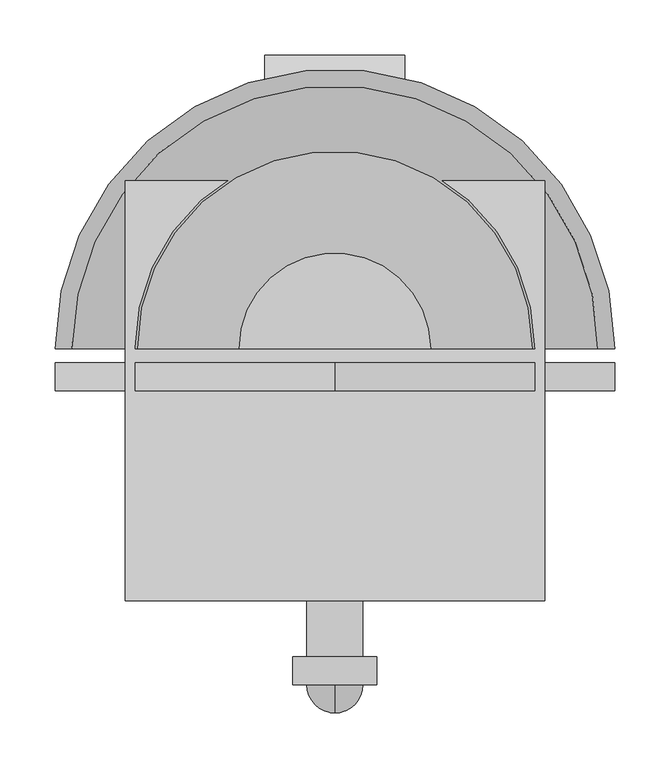
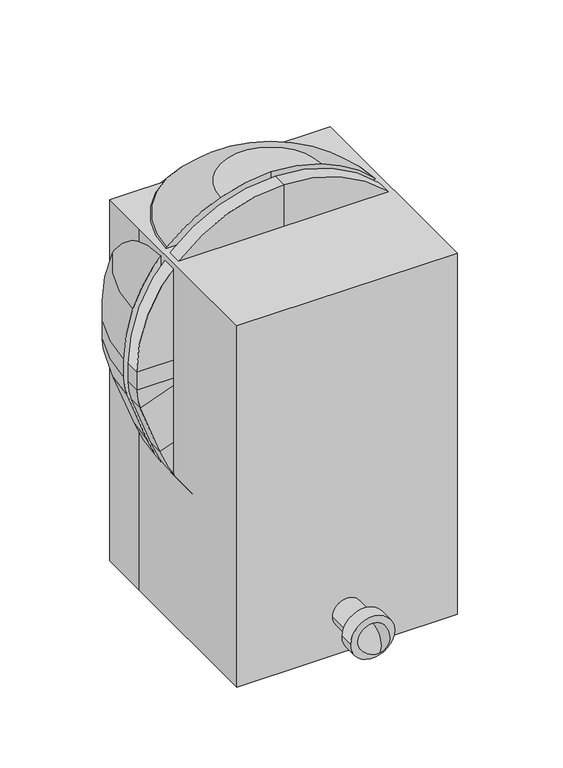
"""IFC4 building model written with IfcOpenShell, lengths in millimetres: proxy geometry, P9050 - Toilet, Wall Hung, Siphon Jet : P9050 - Toilet, Wall Hung, Siphon Jet."""

from ifc_helpers import new_model, si_unit, point, frame, frame_2d, origin, origin_with_axes, place, context, project, spatial, polyline, circle_curve, ellipse_curve, trimmed, segment, composite_curve, outline, extrude, source, transform, mapped, element, save
from ifc_brep_helpers import plane_surface, cylinder_surface, revolved_surface, advanced_brep


def specialty_equipment_177a83fe(model_context):
    return source(origin(), model_context, "Body", "SolidModel", [
        advanced_brep(
        [(-86.8731164, 38.1, 721.2819257), (-179.6051224, 38.1, 662.2051224), (-238.6819257, 38.1, 569.4731164), (-254.0, 38.1, 482.6), (-254.0, 38.1, 449.7148212), (-247.8727703, 38.1, 414.9655747), (-214.4568992, 38.1, 323.1562234), (-180.7778621, 38.1, 258.4593951), (-135.6735798, 38.1, 194.0438043), (-78.7437471, 38.1, 154.1811063), (0.0, 38.1, 133.0817829), (0.0, 38.1, 159.3777978), (-63.2399099, 38.1, 176.3228806), (-120.1697426, 38.1, 216.1855786), (-158.0533758, 38.1, 270.2890139), (-191.7324129, 38.1, 334.9858422), (-224.0045777, 38.1, 423.6528863), (-228.6, 38.1, 449.7148212), (-228.6, 38.1, 482.6), (-214.8137331, 38.1, 560.7858048), (-161.6446102, 38.1, 644.2446102), (-78.1858048, 38.1, 697.4137331), (0.0, 38.1, 711.2), (0.0, 38.1, 736.6), (86.8731164, 38.1, 721.2819257), (78.1858048, 38.1, 697.4137331), (161.6446102, 38.1, 644.2446102), (214.8137331, 38.1, 560.7858048), (228.6, 38.1, 482.6), (228.6, 38.1, 449.7148212), (224.0045777, 38.1, 423.6528863), (191.7324129, 38.1, 334.9858422), (158.0533758, 38.1, 270.2890139), (120.1697426, 38.1, 216.1855786), (63.2399099, 38.1, 176.3228806), (78.7437471, 38.1, 154.1811063), (135.6735798, 38.1, 194.0438043), (180.7778621, 38.1, 258.4593951), (214.4568992, 38.1, 323.1562234), (247.8727703, 38.1, 414.9655747), (254.0, 38.1, 449.7148212), (254.0, 38.1, 482.6), (238.6819257, 38.1, 569.4731164), (179.6051224, 38.1, 662.2051224)],
        [
            (0, 1, circle_curve(frame((0.0, 38.1, 482.6), z_axis=(0.0, -1.0, 0.0), x_axis=(-1.0, 0.0, 0.0)), 254.0)),
            (1, 2, circle_curve(frame((0.0, 38.1, 482.6), z_axis=(0.0, -1.0, 0.0), x_axis=(-1.0, 0.0, 0.0)), 254.0)),
            (2, 3, circle_curve(frame((0.0, 38.1, 482.6), z_axis=(0.0, -1.0, 0.0), x_axis=(-1.0, 0.0, 0.0)), 254.0)),
            (3, 4),
            (4, 5, circle_curve(frame((-152.4, 38.1, 449.7148212), z_axis=(0.0, -1.0, 0.0), x_axis=(-1.0, 0.0, 0.0)), 101.6)),
            (5, 6),
            (6, 7, circle_curve(frame((48.0932191, 38.1, 418.7166514), z_axis=(0.0, -1.0, 0.0), x_axis=(-1.0, 0.0, 0.0)), 279.4)),
            (7, 8),
            (8, 9, circle_curve(frame((-52.4477321, 38.1, 252.3191703), z_axis=(0.0, -1.0, 0.0), x_axis=(-1.0, 0.0, 0.0)), 101.6)),
            (9, 10),
            (10, 11),
            (11, 12),
            (12, 13, circle_curve(frame((-36.9438949, 38.1, 274.4609446), z_axis=(0.0, 1.0, 0.0), x_axis=(-1.0, 0.0, 0.0)), 101.6)),
            (13, 14),
            (14, 15, circle_curve(frame((70.8177054, 38.1, 430.5462703), z_axis=(0.0, 1.0, 0.0), x_axis=(-1.0, 0.0, 0.0)), 279.4)),
            (15, 16),
            (16, 17, circle_curve(frame((-152.4, 38.1, 449.7148212), z_axis=(0.0, 1.0, 0.0), x_axis=(-1.0, 0.0, 0.0)), 76.2)),
            (17, 18),
            (18, 19, circle_curve(frame((0.0, 38.1, 482.6), z_axis=(0.0, 1.0, 0.0), x_axis=(-1.0, 0.0, 0.0)), 228.6)),
            (19, 20, circle_curve(frame((0.0, 38.1, 482.6), z_axis=(0.0, 1.0, 0.0), x_axis=(-1.0, 0.0, 0.0)), 228.6)),
            (20, 21, circle_curve(frame((0.0, 38.1, 482.6), z_axis=(0.0, 1.0, 0.0), x_axis=(-1.0, 0.0, 0.0)), 228.6)),
            (21, 22, circle_curve(frame((0.0, 38.1, 482.6), z_axis=(0.0, 1.0, 0.0), x_axis=(-1.0, 0.0, 0.0)), 228.6)),
            (22, 23),
            (23, 0, circle_curve(frame((0.0, 38.1, 482.6), z_axis=(0.0, -1.0, 0.0), x_axis=(-1.0, 0.0, 0.0)), 254.0)),
            (24, 23, circle_curve(frame((0.0, 38.1, 482.6), z_axis=(0.0, -1.0, 0.0), x_axis=(1.0, 0.0, 0.0)), 254.0)),
            (22, 25, circle_curve(frame((0.0, 38.1, 482.6), z_axis=(0.0, 1.0, 0.0), x_axis=(1.0, 0.0, 0.0)), 228.6)),
            (25, 26, circle_curve(frame((0.0, 38.1, 482.6), z_axis=(0.0, 1.0, 0.0), x_axis=(1.0, 0.0, 0.0)), 228.6)),
            (26, 27, circle_curve(frame((0.0, 38.1, 482.6), z_axis=(0.0, 1.0, 0.0), x_axis=(1.0, 0.0, 0.0)), 228.6)),
            (27, 28, circle_curve(frame((0.0, 38.1, 482.6), z_axis=(0.0, 1.0, 0.0), x_axis=(1.0, 0.0, 0.0)), 228.6)),
            (28, 29),
            (29, 30, circle_curve(frame((152.4, 38.1, 449.7148212), z_axis=(0.0, 1.0, 0.0), x_axis=(1.0, 0.0, 0.0)), 76.2)),
            (30, 31),
            (31, 32, circle_curve(frame((-70.8177054, 38.1, 430.5462703), z_axis=(0.0, 1.0, 0.0), x_axis=(1.0, 0.0, 0.0)), 279.4)),
            (32, 33),
            (33, 34, circle_curve(frame((36.9438949, 38.1, 274.4609446), z_axis=(0.0, 1.0, 0.0), x_axis=(1.0, 0.0, 0.0)), 101.6)),
            (34, 11),
            (10, 35),
            (35, 36, circle_curve(frame((52.4477321, 38.1, 252.3191703), z_axis=(0.0, -1.0, 0.0), x_axis=(1.0, 0.0, 0.0)), 101.6)),
            (36, 37),
            (37, 38, circle_curve(frame((-48.0932191, 38.1, 418.7166514), z_axis=(0.0, -1.0, 0.0), x_axis=(1.0, 0.0, 0.0)), 279.4)),
            (38, 39),
            (39, 40, circle_curve(frame((152.4, 38.1, 449.7148212), z_axis=(0.0, -1.0, 0.0), x_axis=(1.0, 0.0, 0.0)), 101.6)),
            (40, 41),
            (41, 42, circle_curve(frame((0.0, 38.1, 482.6), z_axis=(0.0, -1.0, 0.0), x_axis=(1.0, 0.0, 0.0)), 254.0)),
            (42, 43, circle_curve(frame((0.0, 38.1, 482.6), z_axis=(0.0, -1.0, 0.0), x_axis=(1.0, 0.0, 0.0)), 254.0)),
            (43, 24, circle_curve(frame((0.0, 38.1, 482.6), z_axis=(0.0, -1.0, 0.0), x_axis=(1.0, 0.0, 0.0)), 254.0)),
            (24, 0, circle_curve(frame((0.0, 38.1, 721.2819257), z_axis=(0.0, 0.0, 1.0), x_axis=(-1.0, 0.0, 0.0)), 86.8731164)),
            (21, 25, circle_curve(frame((0.0, 38.1, 697.4137331), z_axis=(0.0, 0.0, -1.0), x_axis=(-1.0, 0.0, 0.0)), 78.1858048)),
            (20, 26, circle_curve(frame((0.0, 38.1, 644.2446102), z_axis=(0.0, 0.0, -1.0), x_axis=(-1.0, 0.0, 0.0)), 161.6446102)),
            (19, 27, circle_curve(frame((0.0, 38.1, 560.7858048), z_axis=(0.0, 0.0, -1.0), x_axis=(-1.0, 0.0, 0.0)), 214.8137331)),
            (18, 28, circle_curve(frame((0.0, 38.1, 482.6), z_axis=(0.0, 0.0, -1.0), x_axis=(-1.0, 0.0, 0.0)), 228.6)),
            (17, 29, circle_curve(frame((0.0, 38.1, 449.7148212), z_axis=(0.0, 0.0, -1.0), x_axis=(-1.0, 0.0, 0.0)), 228.6)),
            (16, 30, circle_curve(frame((0.0, 38.1, 423.6528863), z_axis=(0.0, 0.0, -1.0), x_axis=(-1.0, 0.0, 0.0)), 224.0045777)),
            (15, 31, circle_curve(frame((0.0, 38.1, 334.9858422), z_axis=(0.0, 0.0, -1.0), x_axis=(-1.0, 0.0, 0.0)), 191.7324129)),
            (14, 32, circle_curve(frame((0.0, 38.1, 270.2890139), z_axis=(0.0, 0.0, -1.0), x_axis=(-1.0, 0.0, 0.0)), 158.0533758)),
            (13, 33, circle_curve(frame((0.0, 38.1, 216.1855786), z_axis=(0.0, 0.0, -1.0), x_axis=(-1.0, 0.0, 0.0)), 120.1697426)),
            (12, 34, circle_curve(frame((0.0, 38.1, 176.3228806), z_axis=(0.0, 0.0, -1.0), x_axis=(-1.0, 0.0, 0.0)), 63.2399099)),
            (9, 35, circle_curve(frame((0.0, 38.1, 154.1811063), z_axis=(0.0, 0.0, -1.0), x_axis=(-1.0, 0.0, 0.0)), 78.7437471)),
            (8, 36, circle_curve(frame((0.0, 38.1, 194.0438043), z_axis=(0.0, 0.0, -1.0), x_axis=(-1.0, 0.0, 0.0)), 135.6735798)),
            (7, 37, circle_curve(frame((0.0, 38.1, 258.4593951), z_axis=(0.0, 0.0, -1.0), x_axis=(-1.0, 0.0, 0.0)), 180.7778621)),
            (6, 38, circle_curve(frame((0.0, 38.1, 323.1562234), z_axis=(0.0, 0.0, -1.0), x_axis=(-1.0, 0.0, 0.0)), 214.4568992)),
            (5, 39, circle_curve(frame((0.0, 38.1, 414.9655747), z_axis=(0.0, 0.0, -1.0), x_axis=(-1.0, 0.0, 0.0)), 247.8727703)),
            (4, 40, circle_curve(frame((0.0, 38.1, 449.7148212), z_axis=(0.0, 0.0, -1.0), x_axis=(-1.0, 0.0, 0.0)), 254.0)),
            (3, 41, circle_curve(frame((0.0, 38.1, 482.6), z_axis=(0.0, 0.0, -1.0), x_axis=(-1.0, 0.0, 0.0)), 254.0)),
            (2, 42, circle_curve(frame((0.0, 38.1, 569.4731164), z_axis=(0.0, 0.0, -1.0), x_axis=(-1.0, 0.0, 0.0)), 238.6819257)),
            (1, 43, circle_curve(frame((0.0, 38.1, 662.2051224), z_axis=(0.0, 0.0, -1.0), x_axis=(-1.0, 0.0, 0.0)), 179.6051224)),
        ],
        [
            plane_surface(frame((0.0, 38.1, 841.8102448), z_axis=(0.0, -1.0, 0.0), x_axis=(-1.0, 0.0, 0.0))),
            plane_surface(frame((0.0, 38.1, 841.8102448), z_axis=(0.0, -1.0, 0.0), x_axis=(1.0, 0.0, 0.0))),
            revolved_surface(trimmed(ellipse_curve(frame((0.0, 38.1, 482.6), z_axis=(0.0, 1.0, 0.0), x_axis=(-1.0, 0.0, 0.0)), 254.0, 254.0), [point((-86.8731164, 38.1, 721.2819257))], [point((0.0, 38.1, 736.6))], True, "CARTESIAN"), (0.0, 38.1, 841.8102448), (0.0, 0.0, 1.0)),
            revolved_surface(trimmed(ellipse_curve(frame((0.0, 38.1, 482.6), z_axis=(0.0, -1.0, 0.0), x_axis=(-1.0, 0.0, 0.0)), 228.6, 228.6), [point((0.0, 38.1, 711.2))], [point((-78.1858048, 38.1, 697.4137331))], True, "CARTESIAN"), (0.0, 38.1, 841.8102448), (0.0, 0.0, 1.0)),
            revolved_surface(trimmed(ellipse_curve(frame((0.0, 38.1, 482.6), z_axis=(0.0, -1.0, 0.0), x_axis=(-1.0, 0.0, 0.0)), 228.6, 228.6), [point((-78.1858048, 38.1, 697.4137331))], [point((-161.6446102, 38.1, 644.2446102))], True, "CARTESIAN"), (0.0, 38.1, 841.8102448), (0.0, 0.0, 1.0)),
            revolved_surface(trimmed(ellipse_curve(frame((0.0, 38.1, 482.6), z_axis=(0.0, -1.0, 0.0), x_axis=(-1.0, 0.0, 0.0)), 228.6, 228.6), [point((-161.6446102, 38.1, 644.2446102))], [point((-214.8137331, 38.1, 560.7858048))], True, "CARTESIAN"), (0.0, 38.1, 841.8102448), (0.0, 0.0, 1.0)),
            revolved_surface(trimmed(ellipse_curve(frame((0.0, 38.1, 482.6), z_axis=(0.0, -1.0, 0.0), x_axis=(-1.0, 0.0, 0.0)), 228.6, 228.6), [point((-214.8137331, 38.1, 560.7858048))], [point((-228.6, 38.1, 482.6))], True, "CARTESIAN"), (0.0, 38.1, 841.8102448), (0.0, 0.0, 1.0)),
            revolved_surface(polyline([(-228.6, 38.1, 482.6), (-228.6, 38.1, 449.7148212)]), (0.0, 38.1, 841.8102448), (0.0, 0.0, 1.0)),
            revolved_surface(trimmed(ellipse_curve(frame((-152.4, 38.1, 449.7148212), z_axis=(0.0, -1.0, 0.0), x_axis=(-1.0, 0.0, 0.0)), 76.2, 76.2), [point((-228.6, 38.1, 449.7148212))], [point((-224.0045777, 38.1, 423.6528863))], True, "CARTESIAN"), (0.0, 38.1, 841.8102448), (0.0, 0.0, 1.0)),
            revolved_surface(polyline([(-224.0045777, 38.1, 423.6528863), (-191.7324129, 38.1, 334.9858422)]), (0.0, 38.1, 841.8102448), (0.0, 0.0, 1.0)),
            revolved_surface(trimmed(ellipse_curve(frame((70.8177054, 38.1, 430.5462703), z_axis=(0.0, -1.0, 0.0), x_axis=(-1.0, 0.0, 0.0)), 279.4, 279.4), [point((-191.7324129, 38.1, 334.9858422))], [point((-158.0533758, 38.1, 270.2890139))], True, "CARTESIAN"), (0.0, 38.1, 841.8102448), (0.0, 0.0, 1.0)),
            revolved_surface(polyline([(-158.0533758, 38.1, 270.2890139), (-120.1697426, 38.1, 216.1855786)]), (0.0, 38.1, 841.8102448), (0.0, 0.0, 1.0)),
            revolved_surface(trimmed(ellipse_curve(frame((-36.9438949, 38.1, 274.4609446), z_axis=(0.0, -1.0, 0.0), x_axis=(-1.0, 0.0, 0.0)), 101.6, 101.6), [point((-120.1697426, 38.1, 216.1855786))], [point((-63.2399099, 38.1, 176.3228806))], True, "CARTESIAN"), (0.0, 38.1, 841.8102448), (0.0, 0.0, 1.0)),
            revolved_surface(polyline([(-63.2399099, 38.1, 176.3228806), (0.0, 38.1, 159.3777978)]), (0.0, 38.1, 841.8102448), (0.0, 0.0, 1.0)),
            revolved_surface(polyline([(0.0, 38.1, 133.0817829), (-78.7437471, 38.1, 154.1811063)]), (0.0, 38.1, 841.8102448), (0.0, 0.0, 1.0)),
            revolved_surface(trimmed(ellipse_curve(frame((-52.4477321, 38.1, 252.3191703), z_axis=(0.0, 1.0, 0.0), x_axis=(-1.0, 0.0, 0.0)), 101.6, 101.6), [point((-78.7437471, 38.1, 154.1811063))], [point((-135.6735798, 38.1, 194.0438043))], True, "CARTESIAN"), (0.0, 38.1, 841.8102448), (0.0, 0.0, 1.0)),
            revolved_surface(polyline([(-135.6735798, 38.1, 194.0438043), (-180.7778621, 38.1, 258.4593951)]), (0.0, 38.1, 841.8102448), (0.0, 0.0, 1.0)),
            revolved_surface(trimmed(ellipse_curve(frame((48.0932191, 38.1, 418.7166514), z_axis=(0.0, 1.0, 0.0), x_axis=(-1.0, 0.0, 0.0)), 279.4, 279.4), [point((-180.7778621, 38.1, 258.4593951))], [point((-214.4568992, 38.1, 323.1562234))], True, "CARTESIAN"), (0.0, 38.1, 841.8102448), (0.0, 0.0, 1.0)),
            revolved_surface(polyline([(-214.4568992, 38.1, 323.1562234), (-247.8727703, 38.1, 414.9655747)]), (0.0, 38.1, 841.8102448), (0.0, 0.0, 1.0)),
            revolved_surface(trimmed(ellipse_curve(frame((-152.4, 38.1, 449.7148212), z_axis=(0.0, 1.0, 0.0), x_axis=(-1.0, 0.0, 0.0)), 101.6, 101.6), [point((-247.8727703, 38.1, 414.9655747))], [point((-254.0, 38.1, 449.7148212))], True, "CARTESIAN"), (0.0, 38.1, 841.8102448), (0.0, 0.0, 1.0)),
            cylinder_surface(frame((0.0, 38.1, 841.8102448), z_axis=(0.0, 0.0, 1.0), x_axis=(-1.0, 0.0, 0.0)), 254.0),
            revolved_surface(trimmed(ellipse_curve(frame((0.0, 38.1, 482.6), z_axis=(0.0, 1.0, 0.0), x_axis=(-1.0, 0.0, 0.0)), 254.0, 254.0), [point((-254.0, 38.1, 482.6))], [point((-238.6819257, 38.1, 569.4731164))], True, "CARTESIAN"), (0.0, 38.1, 841.8102448), (0.0, 0.0, 1.0)),
            revolved_surface(trimmed(ellipse_curve(frame((0.0, 38.1, 482.6), z_axis=(0.0, 1.0, 0.0), x_axis=(-1.0, 0.0, 0.0)), 254.0, 254.0), [point((-238.6819257, 38.1, 569.4731164))], [point((-179.6051224, 38.1, 662.2051224))], True, "CARTESIAN"), (0.0, 38.1, 841.8102448), (0.0, 0.0, 1.0)),
            revolved_surface(trimmed(ellipse_curve(frame((0.0, 38.1, 482.6), z_axis=(0.0, 1.0, 0.0), x_axis=(-1.0, 0.0, 0.0)), 254.0, 254.0), [point((-179.6051224, 38.1, 662.2051224))], [point((-86.8731164, 38.1, 721.2819257))], True, "CARTESIAN"), (0.0, 38.1, 841.8102448), (0.0, 0.0, 1.0)),
        ],
        [
            (0, [[1, 2, 3, 4, 5, 6, 7, 8, 9, 10, 11, 12, 13, 14, 15, 16, 17, 18, 19, 20, 21, 22, 23, 24]]),
            (1, [[25, -23, 26, 27, 28, 29, 30, 31, 32, 33, 34, 35, 36, -11, 37, 38, 39, 40, 41, 42, 43, 44, 45, 46]]),
            (2, [[-25, 47, -24]]),
            (3, [[-26, -22, 48]]),
            (4, [[-27, -48, -21, 49]]),
            (5, [[-28, -49, -20, 50]]),
            (6, [[-29, -50, -19, 51]]),
            (7, [[-30, -51, -18, 52]]),
            (8, [[-31, -52, -17, 53]]),
            (9, [[-32, -53, -16, 54]]),
            (10, [[-33, -54, -15, 55]]),
            (11, [[-34, -55, -14, 56]]),
            (12, [[-35, -56, -13, 57]]),
            (13, [[-36, -57, -12]]),
            (14, [[-37, -10, 58]]),
            (15, [[-38, -58, -9, 59]]),
            (16, [[-39, -59, -8, 60]]),
            (17, [[-40, -60, -7, 61]]),
            (18, [[-41, -61, -6, 62]]),
            (19, [[-42, -62, -5, 63]]),
            (20, [[-43, -63, -4, 64]]),
            (21, [[-44, -64, -3, 65]]),
            (22, [[-45, -65, -2, 66]]),
            (23, [[-46, -66, -1, -47]]),
        ],
    ),
        extrude(outline(polyline([(245.0347495, -62.8509631), (194.0438043, -135.6735798), (169.0933226, -110.7230981), (145.0485961, -44.6607552), (145.0485961, 44.6607552), (169.0933226, 110.7230981), (194.0438043, 135.6735798), (245.0347495, 62.8509631), (245.0347495, -62.8509631)])), frame((0.0, 25.4, 0.0), z_axis=(0.0, 1.0, 0.0), x_axis=(0.0, 0.0, 1.0)), (0.0, 0.0, 1.0), 12.7),
        advanced_brep(
        [(-62.8509631, 25.4, 245.0347495), (-62.8509631, 0.0, 245.0347495), (-135.6735798, 0.0, 194.0438043), (-135.6735798, 25.4, 194.0438043), (-180.7778621, 25.4, 258.4593951), (-107.9552454, 25.4, 309.4503403), (-180.7778621, 0.0, 258.4593951), (-107.9552454, 0.0, 309.4503403), (-214.4568992, 25.4, 323.1562234), (-130.9182252, 25.4, 353.5618141), (-214.4568992, 0.0, 323.1562234), (-130.9182252, 0.0, 353.5618141), (-247.8727703, 25.4, 414.9655747), (-164.3340963, 25.4, 445.3711654), (-247.8727703, 0.0, 414.9655747), (-164.3340963, 0.0, 445.3711654), (-254.0, 25.4, 449.7148212), (-165.1, 25.4, 449.7148212), (-254.0, 0.0, 449.7148212), (-165.1, 0.0, 449.7148212), (-254.0, 25.4, 482.6), (-165.1, 25.4, 482.6), (-254.0, 0.0, 482.6), (-165.1, 0.0, 482.6), (0.0, 25.4, 736.6), (0.0, 25.4, 647.7), (0.0, 0.0, 736.6), (0.0, 0.0, 647.7), (254.0, 25.4, 482.6), (165.1, 25.4, 482.6), (254.0, 0.0, 482.6), (165.1, 0.0, 482.6), (254.0, 25.4, 449.7148212), (165.1, 25.4, 449.7148212), (254.0, 0.0, 449.7148212), (165.1, 0.0, 449.7148212), (247.8727703, 25.4, 414.9655747), (164.3340963, 25.4, 445.3711654), (247.8727703, 0.0, 414.9655747), (164.3340963, 0.0, 445.3711654), (214.4568992, 25.4, 323.1562234), (130.9182252, 25.4, 353.5618141), (214.4568992, 0.0, 323.1562234), (130.9182252, 0.0, 353.5618141), (180.7778621, 25.4, 258.4593951), (107.9552454, 25.4, 309.4503403), (180.7778621, 0.0, 258.4593951), (107.9552454, 0.0, 309.4503403), (62.8509631, 25.4, 245.0347495), (135.6735798, 25.4, 194.0438043), (135.6735798, 0.0, 194.0438043), (62.8509631, 0.0, 245.0347495)],
        [
            (0, 1),
            (1, 2),
            (2, 3),
            (3, 0),
            (3, 4),
            (4, 5),
            (5, 0),
            (2, 6),
            (6, 4),
            (1, 7),
            (7, 6),
            (5, 7),
            (8, 9),
            (9, 5, circle_curve(frame((48.0932191, 25.4, 418.7166514), z_axis=(0.0, -1.0, 0.0), x_axis=(-0.81915204428899, 0.0, -0.5735764363510486)), 190.5)),
            (4, 8, circle_curve(frame((48.0932191, 25.4, 418.7166514), z_axis=(0.0, 1.0, 0.0), x_axis=(-0.81915204428899, 0.0, -0.5735764363510486)), 279.4)),
            (10, 8),
            (6, 10, circle_curve(frame((48.0932191, 0.0, 418.7166514), z_axis=(0.0, 1.0, 0.0), x_axis=(-0.81915204428899, 0.0, -0.5735764363510486)), 279.4)),
            (11, 10),
            (7, 11, circle_curve(frame((48.0932191, 0.0, 418.7166514), z_axis=(0.0, 1.0, 0.0), x_axis=(-0.81915204428899, 0.0, -0.5735764363510486)), 190.5)),
            (9, 11),
            (8, 12),
            (12, 13),
            (13, 9),
            (10, 14),
            (14, 12),
            (11, 15),
            (15, 14),
            (13, 15),
            (16, 17),
            (17, 13, circle_curve(frame((-152.4, 25.4, 449.7148212), z_axis=(0.0, -1.0, 0.0), x_axis=(-0.9396926207859067, 0.0, -0.3420201433256736)), 12.7)),
            (12, 16, circle_curve(frame((-152.4, 25.4, 449.7148212), z_axis=(0.0, 1.0, 0.0), x_axis=(-0.9396926207859067, 0.0, -0.3420201433256736)), 101.6)),
            (18, 16),
            (14, 18, circle_curve(frame((-152.4, 0.0, 449.7148212), z_axis=(0.0, 1.0, 0.0), x_axis=(-0.9396926207859067, 0.0, -0.3420201433256736)), 101.6)),
            (19, 18),
            (15, 19, circle_curve(frame((-152.4, 0.0, 449.7148212), z_axis=(0.0, 1.0, 0.0), x_axis=(-0.9396926207859067, 0.0, -0.3420201433256736)), 12.7)),
            (17, 19),
            (16, 20),
            (20, 21),
            (21, 17),
            (18, 22),
            (22, 20),
            (19, 23),
            (23, 22),
            (21, 23),
            (24, 25),
            (25, 21, circle_curve(frame((0.0, 25.4, 482.6), z_axis=(0.0, -1.0, 0.0), x_axis=(-1.0, 0.0, 0.0)), 165.1)),
            (20, 24, circle_curve(frame((0.0, 25.4, 482.6), z_axis=(0.0, 1.0, 0.0), x_axis=(-1.0, 0.0, 0.0)), 254.0)),
            (26, 24),
            (22, 26, circle_curve(frame((0.0, 0.0, 482.6), z_axis=(0.0, 1.0, 0.0), x_axis=(-1.0, 0.0, 0.0)), 254.0)),
            (27, 26),
            (23, 27, circle_curve(frame((0.0, 0.0, 482.6), z_axis=(0.0, 1.0, 0.0), x_axis=(-1.0, 0.0, 0.0)), 165.1)),
            (25, 27),
            (28, 29),
            (29, 25, circle_curve(frame((0.0, 25.4, 482.6), z_axis=(0.0, -1.0, 0.0), x_axis=(0.0, 0.0, 1.0)), 165.1)),
            (24, 28, circle_curve(frame((0.0, 25.4, 482.6), z_axis=(0.0, 1.0, 0.0), x_axis=(0.0, 0.0, 1.0)), 254.0)),
            (30, 28),
            (26, 30, circle_curve(frame((0.0, 0.0, 482.6), z_axis=(0.0, 1.0, 0.0), x_axis=(0.0, 0.0, 1.0)), 254.0)),
            (31, 30),
            (27, 31, circle_curve(frame((0.0, 0.0, 482.6), z_axis=(0.0, 1.0, 0.0), x_axis=(0.0, 0.0, 1.0)), 165.1)),
            (29, 31),
            (28, 32),
            (32, 33),
            (33, 29),
            (30, 34),
            (34, 32),
            (31, 35),
            (35, 34),
            (33, 35),
            (36, 37),
            (37, 33, circle_curve(frame((152.4, 25.4, 449.7148212), z_axis=(0.0, -1.0, 0.0), x_axis=(1.0, 0.0, 0.0)), 12.7)),
            (32, 36, circle_curve(frame((152.4, 25.4, 449.7148212), z_axis=(0.0, 1.0, 0.0), x_axis=(1.0, 0.0, 0.0)), 101.6)),
            (38, 36),
            (34, 38, circle_curve(frame((152.4, 0.0, 449.7148212), z_axis=(0.0, 1.0, 0.0), x_axis=(1.0, 0.0, 0.0)), 101.6)),
            (39, 38),
            (35, 39, circle_curve(frame((152.4, 0.0, 449.7148212), z_axis=(0.0, 1.0, 0.0), x_axis=(1.0, 0.0, 0.0)), 12.7)),
            (37, 39),
            (36, 40),
            (40, 41),
            (41, 37),
            (38, 42),
            (42, 40),
            (39, 43),
            (43, 42),
            (41, 43),
            (44, 45),
            (45, 41, circle_curve(frame((-48.0932191, 25.4, 418.7166514), z_axis=(0.0, -1.0, 0.0), x_axis=(0.9396926207859088, 0.0, -0.34202014332566766)), 190.5)),
            (40, 44, circle_curve(frame((-48.0932191, 25.4, 418.7166514), z_axis=(0.0, 1.0, 0.0), x_axis=(0.9396926207859088, 0.0, -0.34202014332566766)), 279.4)),
            (46, 44),
            (42, 46, circle_curve(frame((-48.0932191, 0.0, 418.7166514), z_axis=(0.0, 1.0, 0.0), x_axis=(0.9396926207859088, 0.0, -0.34202014332566766)), 279.4)),
            (47, 46),
            (43, 47, circle_curve(frame((-48.0932191, 0.0, 418.7166514), z_axis=(0.0, 1.0, 0.0), x_axis=(0.9396926207859088, 0.0, -0.34202014332566766)), 190.5)),
            (45, 47),
            (48, 49),
            (49, 50),
            (50, 51),
            (51, 48),
            (44, 49),
            (48, 45),
            (46, 50),
            (47, 51),
        ],
        [
            plane_surface(frame((-135.6735798, 134.8203184, 194.0438043), z_axis=(0.5735764363510432, 0.0, -0.8191520442889938), x_axis=(0.8191520442889938, 0.0, 0.5735764363510432))),
            plane_surface(frame((-62.8509631, 25.4, 245.0347495), z_axis=(0.0, 1.0, 0.0), x_axis=(-0.5735764363510427, 0.0, 0.8191520442889941))),
            plane_surface(frame((-135.6735798, 25.4, 194.0438043), z_axis=(-0.819152044288994, 0.0, -0.5735764363510429), x_axis=(-0.5735764363510429, 0.0, 0.819152044288994))),
            plane_surface(frame((-135.6735798, 0.0, 194.0438043), z_axis=(0.0, -1.0000000000000002, 0.0), x_axis=(-0.5735764363510432, 0.0, 0.8191520442889939))),
            plane_surface(frame((-62.8509631, 0.0, 245.0347495), z_axis=(0.8191520442889939, 0.0, 0.5735764363510432), x_axis=(-0.5735764363510432, 0.0, 0.8191520442889939))),
            plane_surface(frame((48.0932191, 25.4, 418.7166514), z_axis=(0.0, 1.0, 0.0), x_axis=(-0.81915204428899, 0.0, -0.5735764363510486))),
            cylinder_surface(frame((48.0932191, 38.1, 418.7166514), z_axis=(0.0, -1.0, 0.0), x_axis=(-0.81915204428899, 0.0, -0.5735764363510486)), 279.4),
            plane_surface(frame((48.0932191, 0.0, 418.7166514), z_axis=(0.0, -1.0, 0.0), x_axis=(-0.81915204428899, 0.0, -0.5735764363510486))),
            revolved_surface(polyline([(-107.95524533705259, 0.0, 309.4503402751252), (-107.95524533705259, 25.4, 309.4503402751252)]), (48.0932191, 38.1, 418.7166514), (0.0, -1.0, 0.0)),
            plane_surface(frame((-130.9182252, 25.4, 353.5618141), z_axis=(0.0, 1.0, 0.0), x_axis=(-0.34202014332566844, 0.0, 0.9396926207859085))),
            plane_surface(frame((-214.4568992, 25.4, 323.1562234), z_axis=(-0.9396926207859086, 0.0, -0.3420201433256682), x_axis=(-0.3420201433256682, 0.0, 0.9396926207859086))),
            plane_surface(frame((-214.4568992, 0.0, 323.1562234), z_axis=(0.0, -1.0, 0.0), x_axis=(-0.34202014332566905, 0.0, 0.9396926207859083))),
            plane_surface(frame((-130.9182252, 0.0, 353.5618141), z_axis=(0.9396926207859085, 0.0, 0.34202014332566827), x_axis=(-0.34202014332566827, 0.0, 0.9396926207859085))),
            plane_surface(frame((-152.4, 25.4, 449.7148212), z_axis=(0.0, 1.0, 0.0), x_axis=(-0.9396926207859067, 0.0, -0.3420201433256736))),
            cylinder_surface(frame((-152.4, 38.1, 449.7148212), z_axis=(0.0, -1.0, 0.0), x_axis=(-0.9396926207859067, 0.0, -0.3420201433256736)), 101.6),
            plane_surface(frame((-152.4, 0.0, 449.7148212), z_axis=(0.0, -1.0, 0.0), x_axis=(-0.9396926207859067, 0.0, -0.3420201433256736))),
            revolved_surface(polyline([(-164.334096283981, 0.0, 445.37116537976397), (-164.334096283981, 25.4, 445.37116537976397)]), (-152.4, 38.1, 449.7148212), (0.0, -1.0, 0.0)),
            plane_surface(frame((-165.1, 25.4, 449.7148212), z_axis=(0.0, 1.0, 0.0), x_axis=(0.0, 0.0, 1.0))),
            plane_surface(frame((-254.0, 25.4, 449.7148212), z_axis=(-1.0, 0.0, 0.0), x_axis=(0.0, 0.0, 1.0))),
            plane_surface(frame((-254.0, 0.0, 449.7148212), z_axis=(0.0, -1.0, 0.0), x_axis=(0.0, 0.0, 1.0))),
            plane_surface(frame((-165.1, 0.0, 449.7148212), z_axis=(1.0, 0.0, 0.0), x_axis=(0.0, 0.0, 1.0))),
            plane_surface(frame((0.0, 25.4, 482.6), z_axis=(0.0, 1.0, 0.0), x_axis=(-1.0, 0.0, 0.0))),
            cylinder_surface(frame((0.0, 38.1, 482.6), z_axis=(0.0, -1.0, 0.0), x_axis=(-1.0, 0.0, 0.0)), 254.0),
            plane_surface(frame((0.0, 0.0, 482.6), z_axis=(0.0, -1.0, 0.0), x_axis=(-1.0, 0.0, 0.0))),
            revolved_surface(polyline([(-165.1, 0.0, 482.6), (-165.1, 25.4, 482.6)]), (0.0, 38.1, 482.6), (0.0, -1.0, 0.0)),
            plane_surface(frame((0.0, 25.4, 482.6), z_axis=(0.0, 1.0, 0.0), x_axis=(0.0, 0.0, 1.0))),
            cylinder_surface(frame((0.0, 38.1, 482.6), z_axis=(0.0, -1.0, 0.0), x_axis=(0.0, 0.0, 1.0)), 254.0),
            plane_surface(frame((0.0, 0.0, 482.6), z_axis=(0.0, -1.0, 0.0), x_axis=(0.0, 0.0, 1.0))),
            revolved_surface(polyline([(0.0, 0.0, 647.7), (0.0, 25.4, 647.7)]), (0.0, 38.1, 482.6), (0.0, -1.0, 0.0)),
            plane_surface(frame((165.1, 25.4, 482.6), z_axis=(0.0, 1.0, 0.0), x_axis=(0.0, 0.0, -1.0))),
            plane_surface(frame((254.0, 25.4, 482.6), z_axis=(1.0, 0.0, 0.0), x_axis=(0.0, 0.0, -1.0))),
            plane_surface(frame((254.0, 0.0, 482.6), z_axis=(0.0, -1.0, 0.0), x_axis=(0.0, 0.0, -1.0))),
            plane_surface(frame((165.1, 0.0, 482.6), z_axis=(-1.0, 0.0, 0.0), x_axis=(0.0, 0.0, -1.0))),
            plane_surface(frame((152.4, 25.4, 449.7148212), z_axis=(0.0, 1.0, 0.0), x_axis=(1.0, 0.0, 0.0))),
            cylinder_surface(frame((152.4, 38.1, 449.7148212), z_axis=(0.0, -1.0, 0.0), x_axis=(1.0, 0.0, 0.0)), 101.6),
            plane_surface(frame((152.4, 0.0, 449.7148212), z_axis=(0.0, -1.0, 0.0), x_axis=(1.0, 0.0, 0.0))),
            revolved_surface(polyline([(165.1, 0.0, 449.7148212), (165.1, 25.4, 449.7148212)]), (152.4, 38.1, 449.7148212), (0.0, -1.0, 0.0)),
            plane_surface(frame((164.3340963, 25.4, 445.3711654), z_axis=(0.0, 1.0000000000000002, 0.0), x_axis=(-0.3420201433256679, 0.0, -0.9396926207859088))),
            plane_surface(frame((247.8727703, 25.4, 414.9655747), z_axis=(0.9396926207859088, 0.0, -0.34202014332566794), x_axis=(-0.34202014332566794, 0.0, -0.9396926207859088))),
            plane_surface(frame((247.8727703, 0.0, 414.9655747), z_axis=(0.0, -1.0000000000000002, 0.0), x_axis=(-0.3420201433256676, 0.0, -0.9396926207859089))),
            plane_surface(frame((164.3340963, 0.0, 445.3711654), z_axis=(-0.939692620785909, 0.0, 0.34202014332566727), x_axis=(-0.34202014332566727, 0.0, -0.939692620785909))),
            plane_surface(frame((-48.0932191, 25.4, 418.7166514), z_axis=(0.0, 1.0, 0.0), x_axis=(0.9396926207859088, 0.0, -0.34202014332566766))),
            cylinder_surface(frame((-48.0932191, 38.1, 418.7166514), z_axis=(0.0, -1.0, 0.0), x_axis=(0.9396926207859088, 0.0, -0.34202014332566766)), 279.4),
            plane_surface(frame((-48.0932191, 0.0, 418.7166514), z_axis=(0.0, -1.0, 0.0), x_axis=(0.9396926207859088, 0.0, -0.34202014332566766))),
            revolved_surface(polyline([(130.91822515971563, 0.0, 353.5618140964603), (130.91822515971563, 25.4, 353.5618140964603)]), (-48.0932191, 38.1, 418.7166514), (0.0, -1.0, 0.0)),
            plane_surface(frame((135.6735798, -58.6203184, 194.0438043), z_axis=(-0.5735764363510469, 0.0, -0.8191520442889912), x_axis=(0.8191520442889912, 0.0, -0.5735764363510469))),
            plane_surface(frame((107.9552454, 25.4, 309.4503403), z_axis=(0.0, 1.0, 0.0), x_axis=(-0.5735764363510469, 0.0, -0.8191520442889912))),
            plane_surface(frame((180.7778621, 25.4, 258.4593951), z_axis=(0.8191520442889912, 0.0, -0.5735764363510469), x_axis=(-0.5735764363510469, 0.0, -0.8191520442889912))),
            plane_surface(frame((180.7778621, 0.0, 258.4593951), z_axis=(0.0, -1.0, 0.0), x_axis=(-0.5735764363510466, 0.0, -0.8191520442889915))),
            plane_surface(frame((107.9552454, 0.0, 309.4503403), z_axis=(-0.8191520442889916, 0.0, 0.5735764363510465), x_axis=(-0.5735764363510465, 0.0, -0.8191520442889916))),
        ],
        [
            (0, [[1, 2, 3, 4]]),
            (1, [[5, 6, 7, -4]]),
            (2, [[8, 9, -5, -3]]),
            (3, [[10, 11, -8, -2]]),
            (4, [[-7, 12, -10, -1]]),
            (5, [[13, 14, -6, 15]]),
            (6, [[16, -15, -9, 17]]),
            (7, [[18, -17, -11, 19]]),
            (8, [[20, -19, -12, -14]]),
            (9, [[21, 22, 23, -13]]),
            (10, [[24, 25, -21, -16]]),
            (11, [[26, 27, -24, -18]]),
            (12, [[-23, 28, -26, -20]]),
            (13, [[29, 30, -22, 31]]),
            (14, [[32, -31, -25, 33]]),
            (15, [[34, -33, -27, 35]]),
            (16, [[36, -35, -28, -30]]),
            (17, [[37, 38, 39, -29]]),
            (18, [[40, 41, -37, -32]]),
            (19, [[42, 43, -40, -34]]),
            (20, [[-39, 44, -42, -36]]),
            (21, [[45, 46, -38, 47]]),
            (22, [[48, -47, -41, 49]]),
            (23, [[50, -49, -43, 51]]),
            (24, [[52, -51, -44, -46]]),
            (25, [[53, 54, -45, 55]]),
            (26, [[56, -55, -48, 57]]),
            (27, [[58, -57, -50, 59]]),
            (28, [[60, -59, -52, -54]]),
            (29, [[61, 62, 63, -53]]),
            (30, [[64, 65, -61, -56]]),
            (31, [[66, 67, -64, -58]]),
            (32, [[-63, 68, -66, -60]]),
            (33, [[69, 70, -62, 71]]),
            (34, [[72, -71, -65, 73]]),
            (35, [[74, -73, -67, 75]]),
            (36, [[76, -75, -68, -70]]),
            (37, [[77, 78, 79, -69]]),
            (38, [[80, 81, -77, -72]]),
            (39, [[82, 83, -80, -74]]),
            (40, [[-79, 84, -82, -76]]),
            (41, [[85, 86, -78, 87]]),
            (42, [[88, -87, -81, 89]]),
            (43, [[90, -89, -83, 91]]),
            (44, [[92, -91, -84, -86]]),
            (45, [[93, 94, 95, 96]]),
            (46, [[97, -93, 98, -85]]),
            (47, [[99, -94, -97, -88]]),
            (48, [[100, -95, -99, -90]]),
            (49, [[-98, -96, -100, -92]]),
        ],
    ),
        advanced_brep(
        [(0.0, -266.7, 44.9176912), (0.0, -292.3175826, 70.5352737), (0.0, -266.7, 96.1528563), (0.0, -266.7, 70.5352737)],
        [
            (0, 1, circle_curve(frame((0.0, -266.7, 70.5352737), z_axis=(-1.0, 0.0, 0.0), x_axis=(0.0, 0.0, 1.0)), 25.6175826)),
            (1, 2, circle_curve(frame((0.0, -266.7, 70.5352737), z_axis=(-1.0, 0.0, 0.0), x_axis=(0.0, 0.0, -1.0)), 25.6175826)),
            (2, 0, circle_curve(frame((0.0, -266.7, 70.5352737), z_axis=(0.0, -1.0, 0.0), x_axis=(0.0, 0.0, 1.0)), 25.6175826)),
            (0, 2, circle_curve(frame((0.0, -266.7, 70.5352737), z_axis=(0.0, -1.0, 0.0), x_axis=(0.0, 0.0, 1.0)), 25.6175826)),
            (3, 0),
            (2, 3),
        ],
        [
            revolved_surface(trimmed(ellipse_curve(frame((0.0, -266.7, 70.5352737), z_axis=(-1.0, 0.0, 0.0), x_axis=(0.0, 0.0, -1.0)), 25.6175826, 25.6175826), [point((0.0, -292.3175826, 70.5352737))], [point((0.0, -266.7, 96.1528563))], True, "CARTESIAN"), (0.0, -331.3277273, 70.5352737), (0.0, 1.0, 0.0)),
            plane_surface(frame((0.0, -266.7, 70.5352737), z_axis=(0.0, 1.0, 0.0), x_axis=(0.0, 0.0, 1.0))),
        ],
        [
            (0, [[1, 2, 3]]),
            (0, [[-2, -1, 4]]),
            (1, [[5, -3, 6]]),
            (1, [[-6, -4, -5]]),
        ],
    ),
        extrude(outline(composite_curve([segment(trimmed(circle_curve(frame_2d((70.5352737, 0.0)), 38.1), [point((70.5352737, 38.1))], [point((70.5352737, -38.1))], False, "CARTESIAN"), True, "CONTINUOUS"), segment(trimmed(circle_curve(frame_2d((70.5352737, 0.0)), 38.1), [point((70.5352737, -38.1))], [point((70.5352737, 38.1))], False, "CARTESIAN"), True, "CONTINUOUS")], self_intersect=False)), frame((0.0, -266.7, 0.0), z_axis=(0.0, 1.0, 0.0), x_axis=(0.0, 0.0, 1.0)), (0.0, 0.0, 1.0), 25.4),
        extrude(outline(composite_curve([segment(trimmed(circle_curve(frame_2d((0.0, -163.2113641)), 25.4), [point((25.4, -163.2113641))], [point((-25.4, -163.2113641))], False, "CARTESIAN"), True, "CONTINUOUS"), segment(trimmed(circle_curve(frame_2d((0.0, -163.2113641)), 25.4), [point((-25.4, -163.2113641))], [point((25.4, -163.2113641))], False, "CARTESIAN"), True, "CONTINUOUS")], self_intersect=False)), frame((0.0, 0.0, 37.30625), z_axis=(0.0, 0.0, 1.0), x_axis=(1.0, 0.0, 0.0)), (0.0, 0.0, 1.0), 70.64375),
        extrude(outline(composite_curve([segment(trimmed(circle_curve(frame_2d((70.5352737, 0.0)), 25.4), [point((70.5352737, 25.4))], [point((70.5352737, -25.4))], False, "CARTESIAN"), True, "CONTINUOUS"), segment(trimmed(circle_curve(frame_2d((70.5352737, 0.0)), 25.4), [point((70.5352737, -25.4))], [point((70.5352737, 25.4))], False, "CARTESIAN"), True, "CONTINUOUS")], self_intersect=False)), frame((0.0, -241.3, 0.0), z_axis=(0.0, 1.0, 0.0), x_axis=(0.0, 0.0, 1.0)), (0.0, 0.0, 1.0), 279.4),
        extrude(outline(polyline([(38.1, 152.8037941), (111.703548, 152.8037941), (174.1229337, 196.5103185), (246.9671412, 300.5426282), (304.8, 220.0454017), (304.8, 0.0), (38.1, 0.0), (38.1, 152.8037941)])), frame((-63.5, 0.0, 0.0), z_axis=(1.0, 0.0, 0.0), x_axis=(0.0, 1.0, 0.0)), (0.0, 0.0, 1.0), 127.0),
        extrude(outline(polyline([(-190.5, -190.5), (-190.5, 101.6), (-190.5, 190.5), (190.5, 190.5), (190.5, -190.5), (-190.5, -190.5)])), origin_with_axes(), (0.0, 0.0, 1.0), 660.4),
    ])


if __name__ == "__main__":
    model = new_model("IFC4")
    model_context = context("Model", 3, world=origin())
    ifc_project = project(units=[si_unit("LENGTHUNIT", "METRE", prefix="MILLI")], contexts=[model_context])
    site = spatial("IfcSite", under=ifc_project)
    building = spatial("IfcBuilding", under=site)
    placement = place(None, origin())
    specialty_equipment_shape = specialty_equipment_177a83fe(model_context)
    element("IfcBuildingElementProxy", 1, Name="P9050 - Toilet, Wall Hung, Siphon Jet : P9050 - Toilet, Wall Hung, Siphon Jet", ObjectType="P9050 - Toilet, Wall Hung, Siphon Jet : P9050 - Toilet, Wall Hung, Siphon Jet", at=placement, inside=building, context=model_context, shape_type="MappedRepresentation", body=[
        mapped(specialty_equipment_shape, transform((0.0, 0.0, 0.0), x_axis=(1.0, 0.0, 0.0), y_axis=(0.0, 1.0, 0.0), z_axis=(0.0, 0.0, 1.0))),
    ])
    save(model, "model.ifc")

# Revit data of these elements
# Project information
#   Room Abbreviation = "TLTS2"
#   Room Description = "Toilet/Shower (TLTS2)"
#   Sheets - Total = "5"
#   Project Issue Date = "Issue Date"
#   Project Status = "Project Status"
#   Client Name = "Owner"
#   Project Address = "Enter address here"
#   Project Name = "Project Name"
#   Project Number = "Project Number"
#   Publication Date = "30-Jan-15"
# Type "P9050 - Toilet, Wall Hung, Siphon Jet : P9050 - Toilet, Wall Hung, Siphon Jet"
#   Watts2 = "0"
#   Watts1 = "0"
#   Unit_Issue = "EA"
#   UTIL_6_Misc = "-"
#   UTIL_5_NonMedGas = "-"
#   UTIL_4_MiscGas = "-"
#   UTIL_3_MedGas = "-"
#   UTIL_2_Elec = "-"
#   UTIL_1_WaterDrain = "B"
#   Nomenclature = "Toilet, Wall Hung, Siphon Jet"
#   NSN = "4510"
#   Location [instance default] = ""
#   JSN = "P9050"
#   Fund_Source_VA = "-"
#   Fund_Source_Navy = "-"
#   Fund_Source_Army = "-"
#   Fund_Source_AF = "-"
#   ELEC_Volts2 = "0"
#   ELEC_Volts1 = "0"
#   ELEC_Phase2 = "0"
#   ELEC_Phase1 = "0"
#   ELEC_HertzSwitch = "0"
#   ELEC_HertzDependent = "0"
#   ELEC_Hertz = "0"
#   ELEC_Amps2 = "0"
#   ELEC_Amps1 = "0"
#   DetailDescription = "Siphon jet water closet/ toilet. This unit is wall hung with an elongated bowl, top spud flush valve, seat with open front and check hinge, and carrier. Used throughout the health care facility in restrooms."
#   CAT_VA = "A"
#   CAT_Navy = "A"
#   CAT_IHS = "-"
#   CAT_Army = "A"
#   CAT_AF = "A"
#   BTUperhour = "0"
#   Weight_IP = 60
#   Default Elevation = 1' - 7"
#   DIM_Width_IP = 1' - 3"
#   DIM_Height_IP = 1' - 3"
#   DIM_Depth_IP = 2' - 2"
# Element 1 (IfcBuildingElementProxy, "P9050 - Toilet, Wall Hung, Siphon Jet : P9050 - Toilet, Wall Hung, Siphon Jet")
#   Location = "TLTS2"
#   Materials on its faces: "Laminate - Ivory, Matte", "Porcelain - Ivory", "Metal - Steel, Polished", "EquipSpace"
# Materials
#   "Laminate - Ivory, Matte": class "Miscellaneous", colour RGB 247 247 239, transparency 0
#   "Porcelain - Ivory": class "Unassigned", colour RGB 247 247 239, transparency 0
#   "Metal - Steel, Polished": class "Unassigned", colour RGB 57 57 57, transparency 0
#   "EquipSpace": class "Unassigned", colour RGB 221 217 195, transparency 0.5
